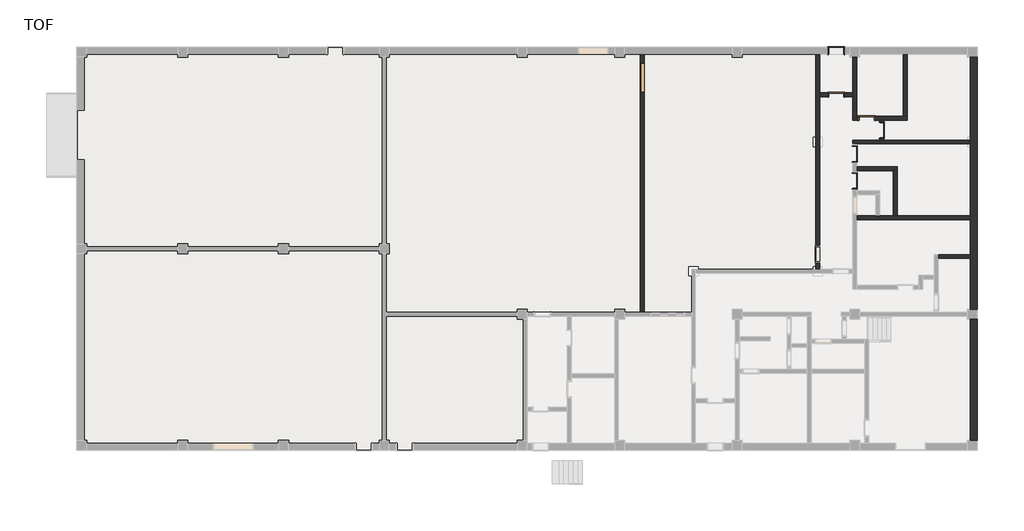
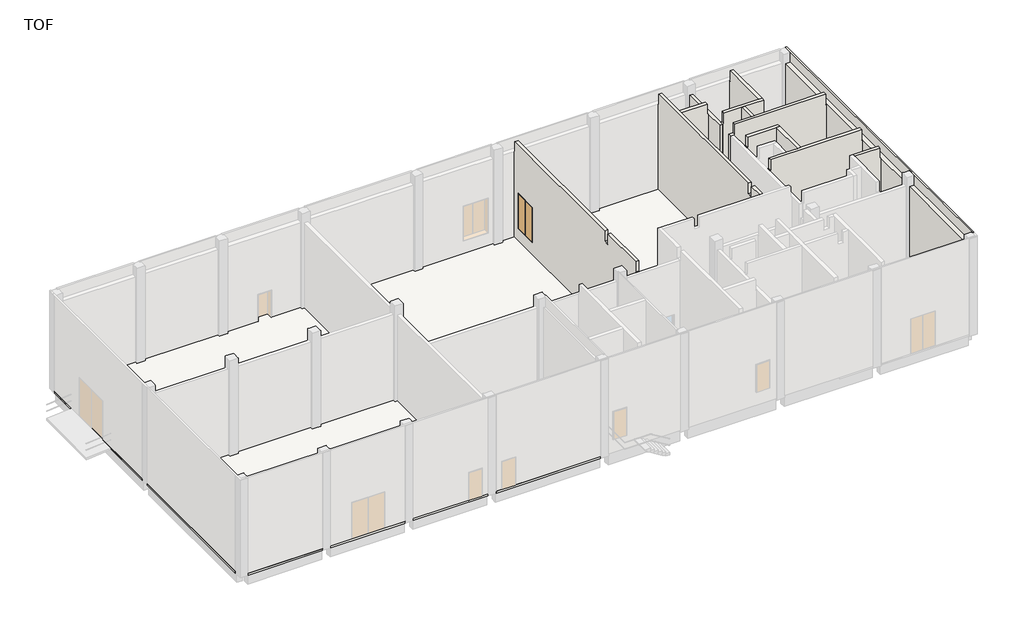
# One storey, part 3 of 5: 13 walls, 7 doors, 2 slabs.
"""IFC4 building model written with IfcOpenShell, lengths in millimetres."""

import ifcopenshell
import ifcopenshell.guid

model = None  # the IFC model being written
_history = None  # IfcOwnerHistory: only IFC2X3 demands one
_inside = {}  # id of a spatial element -> (the spatial element, [elements in it])
_under = {}  # id of a project, library or spatial element -> (it, [spatial elements below it])
_declared = {}  # id of a project -> (the project, [libraries it declares])
_typed = {}  # id of a type object -> (the type object, [elements of that type])
_made_of = {}  # id of a material, layer set ... -> (it, [elements and type objects made of it])


def new_model(schema):
    """Start an empty IFC model of exactly this schema.

    Asked for "IFC4X3", IfcOpenShell would pick the latest addendum, in which some entities
    have other attributes; the version numbers below select the first issue.
    IFC2X3 requires an IfcOwnerHistory on every rooted entity: one is made here for all.
    """
    global model, _history
    if schema == "IFC4X3":
        model = ifcopenshell.file(schema_version=(4, 3, 0, 0))
    else:
        model = ifcopenshell.file(schema=schema)
    _inside.clear()
    _under.clear()
    _declared.clear()
    _typed.clear()
    _made_of.clear()
    _history = None
    if model.schema == "IFC2X3":
        org = make("IfcOrganization", Name="unknown")
        user = make(
            "IfcPersonAndOrganization",
            ThePerson=make("IfcPerson", FamilyName="unknown"),
            TheOrganization=org,
        )
        app = make(
            "IfcApplication",
            ApplicationDeveloper=org,
            Version="unknown",
            ApplicationFullName="unknown",
            ApplicationIdentifier="unknown",
        )
        _history = make(
            "IfcOwnerHistory",
            OwningUser=user,
            OwningApplication=app,
            ChangeAction="ADDED",
            CreationDate=0,
        )
    return model


def make(cls, **values):
    """One entity of the class cls with the attributes given. An attribute that is None is left unset."""
    return model.create_entity(
        cls, **{name: value for name, value in values.items() if value is not None}
    )


def rooted(cls, **values):
    """An entity with a GlobalId (a new one), such as an element, a storey or a relation."""
    return make(cls, GlobalId=ifcopenshell.guid.new(), OwnerHistory=_history, **values)


def si_unit(unit_type, name, prefix=None):
    """IfcSIUnit, for example si_unit("LENGTHUNIT", "METRE", prefix="MILLI")."""
    return make("IfcSIUnit", UnitType=unit_type, Prefix=prefix, Name=name)


def assignment(units):
    """IfcUnitAssignment: the units of a project."""
    return None if units is None else make("IfcUnitAssignment", Units=units)


def point(xyz):
    """IfcCartesianPoint."""
    return None if xyz is None else make("IfcCartesianPoint", Coordinates=xyz)


def direction(xyz):
    """IfcDirection."""
    return None if xyz is None else make("IfcDirection", DirectionRatios=xyz)


def frame(location, z_axis=None, x_axis=None):
    """IfcAxis2Placement3D, a coordinate frame: its origin and axes. An axis left out is left unset."""
    return make(
        "IfcAxis2Placement3D",
        Location=point(location),
        Axis=direction(z_axis),
        RefDirection=direction(x_axis),
    )


def origin():
    """The frame at (0, 0, 0) with its axes left unset."""
    return frame((0.0, 0.0, 0.0))


def origin_with_axes():
    """The frame at (0, 0, 0) with the z axis (0, 0, 1) and the x axis (1, 0, 0) written out."""
    return frame((0.0, 0.0, 0.0), z_axis=(0.0, 0.0, 1.0), x_axis=(1.0, 0.0, 0.0))


def place(relative_to, where):
    """IfcLocalPlacement: puts the frame where relative to a parent placement (None: the world)."""
    return make(
        "IfcLocalPlacement", PlacementRelTo=relative_to, RelativePlacement=where
    )


def context(
    kind, dimensions, precision=None, world=None, true_north=None, identifier=None
):
    """IfcGeometricRepresentationContext, for example the 3D "Model" context."""
    return make(
        "IfcGeometricRepresentationContext",
        ContextIdentifier=identifier,
        ContextType=kind,
        CoordinateSpaceDimension=dimensions,
        Precision=precision,
        WorldCoordinateSystem=world,
        TrueNorth=true_north,
    )


def project(units=None, contexts=None):
    """IfcProject with its units and contexts."""
    return rooted(
        "IfcProject",
        Name="project",
        RepresentationContexts=contexts,
        UnitsInContext=assignment(units),
    )


def spatial(cls, under=None, at=None, **own):
    """A site, building, storey or space (cls), placed at a placement, below another one or the project."""
    s = rooted(cls, ObjectPlacement=at, **own)
    if under is not None:
        _under.setdefault(under.id(), (under, []))[1].append(s)
    return s


def polyline(points):
    """IfcPolyline through the points."""
    return make("IfcPolyline", Points=[point(p) for p in points])


def outline(outer, holes=None, kind="AREA"):
    """IfcArbitraryClosedProfileDef: a profile drawn as a closed curve; with holes, ...WithVoids."""
    if holes is None:
        return make("IfcArbitraryClosedProfileDef", ProfileType=kind, OuterCurve=outer)
    return make(
        "IfcArbitraryProfileDefWithVoids",
        ProfileType=kind,
        OuterCurve=outer,
        InnerCurves=holes,
    )


def extrude(swept, where, along, depth):
    """IfcExtrudedAreaSolid: the profile swept, set in the frame where, extruded along a direction by depth."""
    return make(
        "IfcExtrudedAreaSolid",
        SweptArea=swept,
        Position=where,
        ExtrudedDirection=direction(along),
        Depth=depth,
    )


def faces_of(points, faces, orient=None, outer=None):
    """IfcFace entities. A face is a list of loops; a loop is a list of indices into points, from 0.

    orient and outer hold one flag for each loop. By default every Orientation is true, the
    first loop of a face is its IfcFaceOuterBound and the others are IfcFaceBound.
    """
    made = []
    for i, loops in enumerate(faces):
        bounds = []
        for j, loop in enumerate(loops):
            is_outer = j == 0 if outer is None else outer[i][j]
            bounds.append(
                make(
                    "IfcFaceOuterBound" if is_outer else "IfcFaceBound",
                    Bound=make("IfcPolyLoop", Polygon=[points[k] for k in loop]),
                    Orientation=True if orient is None else orient[i][j],
                )
            )
        made.append(make("IfcFace", Bounds=bounds))
    return made


def faceted_brep(points, faces, orient=None, outer=None, voids=None):
    """IfcFacetedBrep: a solid bounded by flat faces; with voids (closed shells), ...WithVoids."""
    shared = [point(p) for p in points]
    hull = make("IfcClosedShell", CfsFaces=faces_of(shared, faces, orient, outer))
    if voids is None:
        return make("IfcFacetedBrep", Outer=hull)
    return make(
        "IfcFacetedBrepWithVoids",
        Outer=hull,
        Voids=[
            make(cls, CfsFaces=faces_of(shared, fs, o, b)) for cls, fs, o, b in voids
        ],
    )


def shape(context_of_items, identifier, shape_type, items):
    """IfcShapeRepresentation: the items that make up one representation, for example the "Body"."""
    return make(
        "IfcShapeRepresentation",
        ContextOfItems=context_of_items,
        RepresentationIdentifier=identifier,
        RepresentationType=shape_type,
        Items=items,
    )


def source(mapping_origin, context_of_items, identifier, shape_type, items):
    """IfcRepresentationMap: a shape defined once, which mapped items show again and again."""
    return make(
        "IfcRepresentationMap",
        MappingOrigin=mapping_origin,
        MappedRepresentation=shape(context_of_items, identifier, shape_type, items),
    )


def transform(
    local_origin,
    x_axis=None,
    y_axis=None,
    z_axis=None,
    scale=None,
    scale2=None,
    scale3=None,
    uniform=True,
):
    """IfcCartesianTransformationOperator3D, or its non-uniform kind. x_axis, y_axis, z_axis: its Axis1, 2, 3."""
    if uniform:
        return make(
            "IfcCartesianTransformationOperator3D",
            Axis1=direction(x_axis),
            Axis2=direction(y_axis),
            LocalOrigin=point(local_origin),
            Scale=scale,
            Axis3=direction(z_axis),
        )
    return make(
        "IfcCartesianTransformationOperator3DnonUniform",
        Axis1=direction(x_axis),
        Axis2=direction(y_axis),
        LocalOrigin=point(local_origin),
        Scale=scale,
        Axis3=direction(z_axis),
        Scale2=scale2,
        Scale3=scale3,
    )


def mapped(mapping_source, mapping_target):
    """IfcMappedItem: shows the shape of a source again, moved by a transform."""
    return make(
        "IfcMappedItem", MappingSource=mapping_source, MappingTarget=mapping_target
    )


def made_of(thing, what):
    """Note that an element or type object is made of a material, layer set ...; save() writes the relation."""
    if what is not None:
        _made_of.setdefault(what.id(), (what, []))[1].append(thing)
    return thing


def element(
    cls,
    number,
    at=None,
    inside=None,
    cuts=None,
    type_object=None,
    material=None,
    context=None,
    identifier="Body",
    shape_type=None,
    held_by="IfcProductDefinitionShape",
    body=None,
    shapes=None,
    **own,
):
    """One element of the class cls, such as IfcWall. Its Tag is "e" and its number.

    at: its placement. inside: the storey or other place that contains it. cuts: it is an
    opening in that element (IfcRelVoidsElement). A single representation is given by context,
    identifier, shape_type and body (its items); several are given by shapes. held_by: the class
    of the entity that holds the representations. save() writes the other relations.
    """
    e = rooted(cls, Tag="e%d" % number, ObjectPlacement=at, **own)
    if body is not None:
        shapes = [shape(context, identifier, shape_type, body)]
    if shapes is not None:
        e.Representation = make(held_by, Representations=shapes)
    if inside is not None:
        _inside.setdefault(inside.id(), (inside, []))[1].append(e)
    if cuts is not None:
        rooted(
            "IfcRelVoidsElement", RelatingBuildingElement=cuts, RelatedOpeningElement=e
        )
    if type_object is not None:
        _typed.setdefault(type_object.id(), (type_object, []))[1].append(e)
    return made_of(e, material)


def aggregate(whole, parts):
    """IfcRelAggregates: a whole, such as a stair, and the parts it consists of."""
    return rooted("IfcRelAggregates", RelatingObject=whole, RelatedObjects=parts)


def save(model, path):
    """Write the relations noted so far, then the file.

    IfcRelAggregates (storeys below a building ...), IfcRelContainedInSpatialStructure (elements
    in a storey), IfcRelDefinesByType, IfcRelAssociatesMaterial and IfcRelDeclares: one each for
    every whole, place, type object, material and project.
    """
    for whole, parts in _under.values():
        aggregate(whole, parts)
    for where, things in _inside.values():
        rooted(
            "IfcRelContainedInSpatialStructure",
            RelatedElements=things,
            RelatingStructure=where,
        )
    for kind, things in _typed.values():
        rooted("IfcRelDefinesByType", RelatedObjects=things, RelatingType=kind)
    for what, things in _made_of.values():
        rooted("IfcRelAssociatesMaterial", RelatedObjects=things, RelatingMaterial=what)
    for by, libraries in _declared.values():
        rooted("IfcRelDeclares", RelatingContext=by, RelatedDefinitions=libraries)
    model.write(path)


def double_door_steel_474d71af(model_context):
    return source(origin(), model_context, "Body", "SolidModel", [
        extrude(outline(polyline([(880.0, 77.0), (0.0, 77.0), (0.0, 117.0), (880.0, 117.0), (880.0, 77.0)])), frame((0.0, 0.0, 20.0), z_axis=(0.0, 0.0, 1.0), x_axis=(1.0, 0.0, 0.0)), (0.0, 0.0, 1.0), 2660.0),
        extrude(outline(polyline([(0.0, 77.0), (-880.0, 77.0), (-880.0, 117.0), (0.0, 117.0), (0.0, 77.0)])), frame((0.0, 0.0, 20.0), z_axis=(0.0, 0.0, 1.0), x_axis=(1.0, 0.0, 0.0)), (0.0, 0.0, 1.0), 2660.0),
        faceted_brep([(900.0, -117.0, 2700.0), (900.0, 117.0, 2700.0), (-900.0, 117.0, 2700.0), (-900.0, -117.0, 2700.0), (865.0, 77.0, 2665.0), (865.0, -117.0, 2665.0), (-865.0, -117.0, 2665.0), (-865.0, 77.0, 2665.0), (880.0, 117.0, 2680.0), (880.0, 77.0, 2680.0), (-880.0, 77.0, 2680.0), (-880.0, 117.0, 2680.0), (-900.0, 117.0, 0.0), (-900.0, -117.0, 0.0), (-865.0, -117.0, 35.0), (-865.0, 77.0, 35.0), (-880.0, 77.0, 20.0), (-880.0, 117.0, 20.0), (900.0, 117.0, 0.0), (880.0, 117.0, 20.0), (900.0, -117.0, 0.0), (865.0, -117.0, 35.0), (865.0, 77.0, 35.0), (880.0, 77.0, 20.0)], [[[0, 1, 2, 3]], [[4, 5, 6, 7]], [[8, 9, 10, 11]], [[3, 2, 12, 13]], [[7, 6, 14, 15]], [[11, 10, 16, 17]], [[18, 12, 2, 1], [8, 11, 17, 19]], [[13, 12, 18, 20]], [[0, 3, 13, 20], [21, 14, 6, 5]], [[15, 14, 21, 22]], [[23, 16, 10, 9], [4, 7, 15, 22]], [[17, 16, 23, 19]], [[20, 18, 1, 0]], [[22, 21, 5, 4]], [[19, 23, 9, 8]]]),
    ])


def single_door_steel_cad2a4f8(model_context):
    return source(origin(), model_context, "Body", "SolidModel", [
        extrude(outline(polyline([(470.0, -245.0), (-470.0, -245.0), (-470.0, -210.0), (470.0, -210.0), (470.0, -245.0)])), origin_with_axes(), (0.0, 0.0, 1.0), 2120.0),
        faceted_brep([(470.0, -245.0, 0.0), (470.0, -210.0, 0.0), (450.0, -210.0, 0.0), (450.0, 210.0, 0.0), (470.0, 210.0, 0.0), (470.0, 245.0, 0.0), (500.0, 245.0, 0.0), (500.0, -245.0, 0.0), (500.0, -245.0, 2150.0), (-500.0, -245.0, 2150.0), (-500.0, -245.0, 0.0), (-470.0, -245.0, 0.0), (-470.0, -245.0, 2120.0), (470.0, -245.0, 2120.0), (500.0, 245.0, 2150.0), (470.0, 245.0, 2120.0), (-470.0, 245.0, 2120.0), (-470.0, 245.0, 0.0), (-500.0, 245.0, 0.0), (-500.0, 245.0, 2150.0), (470.0, 210.0, 2120.0), (450.0, 210.0, 2100.0), (-450.0, 210.0, 2100.0), (-450.0, 210.0, 0.0), (-470.0, 210.0, 0.0), (-470.0, 210.0, 2120.0), (450.0, -210.0, 2100.0), (470.0, -210.0, 2120.0), (-470.0, -210.0, 2120.0), (-470.0, -210.0, 0.0), (-450.0, -210.0, 0.0), (-450.0, -210.0, 2100.0)], [[[0, 1, 2, 3, 4, 5, 6, 7]], [[7, 8, 9, 10, 11, 12, 13, 0]], [[6, 14, 8, 7]], [[5, 15, 16, 17, 18, 19, 14, 6]], [[4, 20, 15, 5]], [[3, 21, 22, 23, 24, 25, 20, 4]], [[2, 26, 21, 3]], [[1, 27, 28, 29, 30, 31, 26, 2]], [[0, 13, 27, 1]], [[12, 11, 29, 28]], [[11, 10, 18, 17, 24, 23, 30, 29]], [[19, 18, 10, 9]], [[25, 24, 17, 16]], [[31, 30, 23, 22]], [[14, 19, 9, 8]], [[20, 25, 16, 15]], [[26, 31, 22, 21]], [[13, 12, 28, 27]]]),
    ])


def single_door_steel_d38beafa(model_context):
    return source(origin(), model_context, "Body", "SolidModel", [
        extrude(outline(polyline([(470.0, 147.0), (470.0, 112.0), (-470.0, 112.0), (-470.0, 147.0), (470.0, 147.0)])), origin_with_axes(), (0.0, 0.0, 1.0), 2120.0),
        faceted_brep([(470.0, 147.0, 0.0), (500.0, 147.0, 0.0), (500.0, -147.0, 0.0), (470.0, -147.0, 0.0), (470.0, -112.0, 0.0), (450.0, -112.0, 0.0), (450.0, 112.0, 0.0), (470.0, 112.0, 0.0), (470.0, 147.0, 2120.0), (-470.0, 147.0, 2120.0), (-470.0, 147.0, 0.0), (-500.0, 147.0, 0.0), (-500.0, 147.0, 2150.0), (500.0, 147.0, 2150.0), (500.0, -147.0, 2150.0), (-500.0, -147.0, 2150.0), (-500.0, -147.0, 0.0), (-470.0, -147.0, 0.0), (-470.0, -147.0, 2120.0), (470.0, -147.0, 2120.0), (470.0, -112.0, 2120.0), (-470.0, -112.0, 2120.0), (-470.0, -112.0, 0.0), (-450.0, -112.0, 0.0), (-450.0, -112.0, 2100.0), (450.0, -112.0, 2100.0), (450.0, 112.0, 2100.0), (-450.0, 112.0, 2100.0), (-450.0, 112.0, 0.0), (-470.0, 112.0, 0.0), (-470.0, 112.0, 2120.0), (470.0, 112.0, 2120.0)], [[[0, 1, 2, 3, 4, 5, 6, 7]], [[1, 0, 8, 9, 10, 11, 12, 13]], [[2, 1, 13, 14]], [[3, 2, 14, 15, 16, 17, 18, 19]], [[4, 3, 19, 20]], [[5, 4, 20, 21, 22, 23, 24, 25]], [[6, 5, 25, 26]], [[7, 6, 26, 27, 28, 29, 30, 31]], [[0, 7, 31, 8]], [[9, 30, 29, 10]], [[10, 29, 28, 23, 22, 17, 16, 11]], [[15, 12, 11, 16]], [[21, 18, 17, 22]], [[27, 24, 23, 28]], [[14, 13, 12, 15]], [[20, 19, 18, 21]], [[26, 25, 24, 27]], [[8, 31, 30, 9]]]),
    ])


def single_door_steel_221a647d(model_context):
    return source(origin(), model_context, "Body", "SolidModel", [
        extrude(outline(polyline([(470.0, -147.0), (-470.0, -147.0), (-470.0, -112.0), (470.0, -112.0), (470.0, -147.0)])), origin_with_axes(), (0.0, 0.0, 1.0), 2120.0),
        faceted_brep([(470.0, -147.0, 0.0), (470.0, -112.0, 0.0), (450.0, -112.0, 0.0), (450.0, 112.0, 0.0), (470.0, 112.0, 0.0), (470.0, 147.0, 0.0), (500.0, 147.0, 0.0), (500.0, -147.0, 0.0), (500.0, -147.0, 2150.0), (-500.0, -147.0, 2150.0), (-500.0, -147.0, 0.0), (-470.0, -147.0, 0.0), (-470.0, -147.0, 2120.0), (470.0, -147.0, 2120.0), (500.0, 147.0, 2150.0), (470.0, 147.0, 2120.0), (-470.0, 147.0, 2120.0), (-470.0, 147.0, 0.0), (-500.0, 147.0, 0.0), (-500.0, 147.0, 2150.0), (470.0, 112.0, 2120.0), (450.0, 112.0, 2100.0), (-450.0, 112.0, 2100.0), (-450.0, 112.0, 0.0), (-470.0, 112.0, 0.0), (-470.0, 112.0, 2120.0), (450.0, -112.0, 2100.0), (470.0, -112.0, 2120.0), (-470.0, -112.0, 2120.0), (-470.0, -112.0, 0.0), (-450.0, -112.0, 0.0), (-450.0, -112.0, 2100.0)], [[[0, 1, 2, 3, 4, 5, 6, 7]], [[7, 8, 9, 10, 11, 12, 13, 0]], [[6, 14, 8, 7]], [[5, 15, 16, 17, 18, 19, 14, 6]], [[4, 20, 15, 5]], [[3, 21, 22, 23, 24, 25, 20, 4]], [[2, 26, 21, 3]], [[1, 27, 28, 29, 30, 31, 26, 2]], [[0, 13, 27, 1]], [[12, 11, 29, 28]], [[11, 10, 18, 17, 24, 23, 30, 29]], [[19, 18, 10, 9]], [[25, 24, 17, 16]], [[31, 30, 23, 22]], [[14, 19, 9, 8]], [[20, 25, 16, 15]], [[26, 31, 22, 21]], [[13, 12, 28, 27]]]),
    ])


model = new_model("IFC4")

# Units and contexts
model_context = context("Model", 3, world=origin())
ifc_project = project(units=[si_unit("LENGTHUNIT", "METRE", prefix="MILLI")], contexts=[model_context])

# Site, building, storey
site = spatial("IfcSite", under=ifc_project)
building = spatial("IfcBuilding", under=site)
storey = spatial("IfcBuildingStorey", under=building, Name="TOF", Elevation=150.0)

# Doors
placement = place(None, origin())
double_door_steel_shape = double_door_steel_474d71af(model_context)
element("IfcDoor", 1, ObjectType="Double Door_Steel", at=placement, inside=storey, context=model_context, shape_type="MappedRepresentation", body=[
    mapped(double_door_steel_shape, transform((33274.7, 22486.5208589, 1150.0), x_axis=(0.0, 1.0, 0.0), y_axis=(-1.0, 0.0, 0.0), z_axis=(0.0, 0.0, 1.0))),
])
single_door_steel_shape = single_door_steel_cad2a4f8(model_context)
element("IfcDoor", 2, ObjectType="Single Door_Steel", at=placement, inside=storey, context=model_context, shape_type="MappedRepresentation", body=[
    mapped(single_door_steel_shape, transform((44824.7, 24101.5208589, 1150.0), x_axis=(-1.0, 0.0, 0.0), y_axis=(0.0, -1.0, 0.0), z_axis=(0.0, 0.0, 1.0))),
])
single_door_steel_2_shape = single_door_steel_d38beafa(model_context)
element("IfcDoor", 3, ObjectType="Single Door_Steel", at=placement, inside=storey, context=model_context, shape_type="MappedRepresentation", body=[
    mapped(single_door_steel_2_shape, transform((46641.7, 20066.5208589, 1150.0), x_axis=(1.0, 0.0, 0.0), y_axis=(0.0, 1.0, 0.0), z_axis=(0.0, 0.0, 1.0))),
])
element("IfcDoor", 4, ObjectType="Single Door_Steel", at=placement, inside=storey, context=model_context, shape_type="MappedRepresentation", body=[
    mapped(single_door_steel_2_shape, transform((45924.7, 17949.5208589, 1150.0), x_axis=(0.0, -1.0, 0.0), y_axis=(1.0, 0.0, 0.0), z_axis=(0.0, 0.0, 1.0))),
])
element("IfcDoor", 5, ObjectType="Single Door_Steel", at=placement, inside=storey, context=model_context, shape_type="MappedRepresentation", body=[
    mapped(single_door_steel_2_shape, transform((45924.7, 16350.3721317, 1150.0), x_axis=(0.0, -1.0, 0.0), y_axis=(1.0, 0.0, 0.0), z_axis=(0.0, 0.0, 1.0))),
])
single_door_steel_3_shape = single_door_steel_221a647d(model_context)
element("IfcDoor", 6, ObjectType="Single Door_Steel", at=placement, inside=storey, context=model_context, shape_type="MappedRepresentation", body=[
    mapped(single_door_steel_3_shape, transform((44824.7, 21469.5208589, 1150.0), x_axis=(-1.0, 0.0, 0.0), y_axis=(0.0, -1.0, 0.0), z_axis=(0.0, 0.0, 1.0))),
])
element("IfcDoor", 7, ObjectType="Single Door_Steel", at=placement, inside=storey, context=model_context, shape_type="MappedRepresentation", body=[
    mapped(single_door_steel_3_shape, transform((47541.7, 19366.5208589, 1150.0), x_axis=(0.0, 1.0, 0.0), y_axis=(-1.0, 0.0, 0.0), z_axis=(0.0, 0.0, 1.0))),
])

# Slabs
element("IfcSlab", 8, at=placement, inside=storey, context=model_context, shape_type="Brep", body=[
    faceted_brep([(224.7, 12316.5208589, 50.0), (224.7, 12616.5208589, 50.0), (124.7, 12616.5208589, 50.0), (-275.3, 12616.5208589, 50.0), (-375.3, 12616.5208589, 50.0), (-375.3, 23716.5208589, 50.0), (-275.3, 23716.5208589, 50.0), (124.7, 23716.5208589, 50.0), (224.7, 23716.5208589, 50.0), (224.7, 23816.5208589, 50.0), (224.7, 24216.5208589, 50.0), (224.7, 24316.5208589, 50.0), (5624.7, 24316.5208589, 50.0), (5624.7, 24216.5208589, 50.0), (5624.7, 23816.5208589, 50.0), (5624.7, 23716.5208589, 50.0), (6224.7, 23716.5208589, 50.0), (6224.7, 23816.5208589, 50.0), (6224.7, 24216.5208589, 50.0), (6224.7, 24316.5208589, 50.0), (11624.7, 24316.5208589, 50.0), (11624.7, 24216.5208589, 50.0), (11624.7, 23816.5208589, 50.0), (11624.7, 23716.5208589, 50.0), (12224.7, 23716.5208589, 50.0), (12224.7, 23816.5208589, 50.0), (12224.7, 24216.5208589, 50.0), (12224.7, 24316.5208589, 50.0), (17624.7, 24316.5208589, 50.0), (17624.7, 24216.5208589, 50.0), (17624.7, 23816.5208589, 50.0), (17624.7, 23716.5208589, 50.0), (18224.7, 23716.5208589, 50.0), (18224.7, 23816.5208589, 50.0), (18224.7, 24216.5208589, 50.0), (18224.7, 24316.5208589, 50.0), (25824.7, 24316.5208589, 50.0), (25824.7, 24216.5208589, 50.0), (25824.7, 23816.5208589, 50.0), (25824.7, 23716.5208589, 50.0), (26424.7, 23716.5208589, 50.0), (26424.7, 23816.5208589, 50.0), (26424.7, 24216.5208589, 50.0), (26424.7, 24316.5208589, 50.0), (31624.7, 24316.5208589, 50.0), (31624.7, 24216.5208589, 50.0), (31624.7, 23816.5208589, 50.0), (31624.7, 23716.5208589, 50.0), (32224.7, 23716.5208589, 50.0), (32224.7, 23816.5208589, 50.0), (32224.7, 24216.5208589, 50.0), (32224.7, 24316.5208589, 50.0), (38624.7, 24316.5208589, 50.0), (38624.7, 24216.5208589, 50.0), (38624.7, 23816.5208589, 50.0), (38624.7, 23716.5208589, 50.0), (39224.7, 23716.5208589, 50.0), (39224.7, 23816.5208589, 50.0), (39224.7, 24216.5208589, 50.0), (39224.7, 24316.5208589, 50.0), (43724.7, 24316.5208589, 50.0), (43724.7, 24216.5208589, 50.0), (43724.7, 23816.5208589, 50.0), (43724.7, 18966.5208589, 50.0), (43424.7, 18966.5208589, 50.0), (43424.7, 18366.5208589, 50.0), (43724.7, 18366.5208589, 50.0), (43724.7, 11266.5208589, 50.0), (43424.7, 11266.5208589, 50.0), (43424.7, 10966.5208589, 50.0), (36624.7, 10966.5208589, 50.0), (36624.7, 11266.5208589, 50.0), (36024.7, 11266.5208589, 50.0), (36024.7, 10666.5208589, 50.0), (36324.7, 10666.5208589, 50.0), (36324.7, 8416.5208589, 50.0), (32224.7, 8416.5208589, 50.0), (32224.7, 8716.5208589, 50.0), (31624.7, 8716.5208589, 50.0), (31624.7, 8416.5208589, 50.0), (26424.7, 8416.5208589, 50.0), (26424.7, 8716.5208589, 50.0), (25824.7, 8716.5208589, 50.0), (25824.7, 8416.5208589, 50.0), (17924.7, 8416.5208589, 50.0), (17924.7, 12016.5208589, 50.0), (18224.7, 12016.5208589, 50.0), (18224.7, 12616.5208589, 50.0), (17624.7, 12616.5208589, 50.0), (17624.7, 12316.5208589, 50.0), (12224.7, 12316.5208589, 50.0), (12224.7, 12616.5208589, 50.0), (11624.7, 12616.5208589, 50.0), (11624.7, 12316.5208589, 50.0), (6224.7, 12316.5208589, 50.0), (6224.7, 12616.5208589, 50.0), (5624.7, 12616.5208589, 50.0), (5624.7, 12316.5208589, 50.0), (5624.7, 12616.5208589, 200.0), (6224.7, 12616.5208589, 200.0), (6224.7, 12433.5208589, 200.0), (11624.7, 12433.5208589, 200.0), (11624.7, 12616.5208589, 200.0), (12224.7, 12616.5208589, 200.0), (12224.7, 12433.5208589, 200.0), (17624.7, 12433.5208589, 200.0), (17624.7, 12616.5208589, 200.0), (17807.7, 12616.5208589, 200.0), (17807.7, 23716.5208589, 200.0), (17624.7, 23716.5208589, 200.0), (17624.7, 23886.5208589, 200.0), (15507.7, 23886.5208589, 200.0), (15507.7, 24316.5208589, 200.0), (14507.7, 24316.5208589, 200.0), (14507.7, 23886.5208589, 200.0), (12224.7, 23886.5208589, 200.0), (12224.7, 23716.5208589, 200.0), (11624.7, 23716.5208589, 200.0), (11624.7, 23886.5208589, 200.0), (6224.7, 23886.5208589, 200.0), (6224.7, 23716.5208589, 200.0), (5624.7, 23716.5208589, 200.0), (5624.7, 23886.5208589, 200.0), (224.7, 23886.5208589, 200.0), (224.7, 23716.5208589, 200.0), (54.7, 23716.5208589, 200.0), (54.7, 20586.5208589, 200.0), (-375.3, 20586.5208589, 200.0), (-375.3, 17586.5208589, 200.0), (54.7, 17586.5208589, 200.0), (54.7, 12616.5208589, 200.0), (224.7, 12616.5208589, 200.0), (224.7, 12433.5208589, 200.0), (5624.7, 12433.5208589, 200.0), (18224.7, 12616.5208589, 200.0), (18224.7, 12016.5208589, 200.0), (18041.7, 12016.5208589, 200.0), (18041.7, 8533.5208589, 200.0), (25824.7, 8533.5208589, 200.0), (25824.7, 8716.5208589, 200.0), (26424.7, 8716.5208589, 200.0), (26424.7, 8533.5208589, 200.0), (31624.7, 8533.5208589, 200.0), (31624.7, 8716.5208589, 200.0), (32224.7, 8716.5208589, 200.0), (32224.7, 8533.5208589, 200.0), (33157.7, 8533.5208589, 200.0), (33157.7, 23886.5208589, 200.0), (32224.7, 23886.5208589, 200.0), (32224.7, 23716.5208589, 200.0), (31624.7, 23716.5208589, 200.0), (31624.7, 23886.5208589, 200.0), (26424.7, 23886.5208589, 200.0), (26424.7, 23716.5208589, 200.0), (25824.7, 23716.5208589, 200.0), (25824.7, 23886.5208589, 200.0), (18224.7, 23886.5208589, 200.0), (18224.7, 23716.5208589, 200.0), (18041.7, 23716.5208589, 200.0), (18041.7, 12616.5208589, 200.0), (39224.7, 23716.5208589, 200.0), (38624.7, 23716.5208589, 200.0), (38624.7, 23886.5208589, 200.0), (33391.7, 23886.5208589, 200.0), (33391.7, 8533.5208589, 200.0), (36207.7, 8533.5208589, 200.0), (36207.7, 8416.5208589, 200.0), (36324.7, 8416.5208589, 200.0), (36324.7, 10666.5208589, 200.0), (36024.7, 10666.5208589, 200.0), (36024.7, 11266.5208589, 200.0), (36624.7, 11266.5208589, 200.0), (36624.7, 11083.5208589, 200.0), (43424.7, 11083.5208589, 200.0), (43424.7, 11266.5208589, 200.0), (43607.7, 11266.5208589, 200.0), (43607.7, 18366.5208589, 200.0), (43424.7, 18366.5208589, 200.0), (43424.7, 18966.5208589, 200.0), (43607.7, 18966.5208589, 200.0), (43607.7, 23886.5208589, 200.0), (39224.7, 23886.5208589, 200.0), (-375.3, 12616.5208589, 150.0), (-375.3, 17586.5208589, 150.0), (-375.3, 20586.5208589, 150.0), (-375.3, 23716.5208589, 150.0), (224.7, 24316.5208589, 150.0), (5624.7, 24316.5208589, 150.0), (6224.7, 24316.5208589, 150.0), (11624.7, 24316.5208589, 150.0), (12224.7, 24316.5208589, 150.0), (14507.7, 24316.5208589, 150.0), (15507.7, 24316.5208589, 150.0), (17624.7, 24316.5208589, 150.0), (18224.7, 24316.5208589, 150.0), (25824.7, 24316.5208589, 150.0), (26424.7, 24316.5208589, 150.0), (31624.7, 24316.5208589, 150.0), (39224.7, 24316.5208589, 150.0), (43724.7, 24316.5208589, 150.0), (32224.7, 24316.5208589, 150.0), (38624.7, 24316.5208589, 150.0), (43724.7, 18366.5208589, 150.0), (43724.7, 11266.5208589, 150.0), (43724.7, 24216.5208589, 150.0), (43724.7, 23816.5208589, 150.0), (43724.7, 18966.5208589, 150.0), (43424.7, 10966.5208589, 150.0), (36624.7, 10966.5208589, 150.0), (36207.7, 8416.5208589, 150.0), (32224.7, 8416.5208589, 150.0), (25824.7, 8416.5208589, 150.0), (17924.7, 8416.5208589, 150.0), (31624.7, 8416.5208589, 150.0), (26424.7, 8416.5208589, 150.0), (17924.7, 12016.5208589, 150.0), (5624.7, 12316.5208589, 150.0), (224.7, 12316.5208589, 150.0), (11624.7, 12316.5208589, 150.0), (6224.7, 12316.5208589, 150.0), (17624.7, 12316.5208589, 150.0), (12224.7, 12316.5208589, 150.0), (224.7, 12433.5208589, 150.0), (54.7, 12616.5208589, 150.0), (6224.7, 12433.5208589, 150.0), (5624.7, 12433.5208589, 150.0), (12224.7, 12433.5208589, 150.0), (11624.7, 12433.5208589, 150.0), (18041.7, 12016.5208589, 150.0), (17624.7, 12433.5208589, 150.0), (18041.7, 12616.5208589, 150.0), (17807.7, 12616.5208589, 150.0), (224.7, 23886.5208589, 150.0), (54.7, 23716.5208589, 150.0), (6224.7, 23886.5208589, 150.0), (5624.7, 23886.5208589, 150.0), (12224.7, 23886.5208589, 150.0), (11624.7, 23886.5208589, 150.0), (18224.7, 23886.5208589, 150.0), (17807.7, 23716.5208589, 150.0), (18041.7, 23716.5208589, 150.0), (17624.7, 23886.5208589, 150.0), (26424.7, 23886.5208589, 150.0), (25824.7, 23886.5208589, 150.0), (32224.7, 23886.5208589, 150.0), (31624.7, 23886.5208589, 150.0), (39224.7, 23886.5208589, 150.0), (38624.7, 23886.5208589, 150.0), (26424.7, 8533.5208589, 150.0), (25824.7, 8533.5208589, 150.0), (32224.7, 8533.5208589, 150.0), (31624.7, 8533.5208589, 150.0), (36624.7, 11083.5208589, 150.0), (43424.7, 11083.5208589, 150.0), (43607.7, 11266.5208589, 150.0), (43607.7, 18366.5208589, 150.0), (43607.7, 18966.5208589, 150.0), (33157.7, 23886.5208589, 150.0), (43607.7, 23886.5208589, 150.0), (33391.7, 23886.5208589, 150.0), (15507.7, 23886.5208589, 150.0), (14507.7, 23886.5208589, 150.0), (18041.7, 8533.5208589, 150.0), (33157.7, 8533.5208589, 150.0), (36207.7, 8533.5208589, 150.0), (33391.7, 8533.5208589, 150.0), (54.7, 20586.5208589, 150.0), (54.7, 17586.5208589, 150.0)], [[[0, 1, 2, 3, 4, 5, 6, 7, 8, 9, 10, 11, 12, 13, 14, 15, 16, 17, 18, 19, 20, 21, 22, 23, 24, 25, 26, 27, 28, 29, 30, 31, 32, 33, 34, 35, 36, 37, 38, 39, 40, 41, 42, 43, 44, 45, 46, 47, 48, 49, 50, 51, 52, 53, 54, 55, 56, 57, 58, 59, 60, 61, 62, 63, 64, 65, 66, 67, 68, 69, 70, 71, 72, 73, 74, 75, 76, 77, 78, 79, 80, 81, 82, 83, 84, 85, 86, 87, 88, 89, 90, 91, 92, 93, 94, 95, 96, 97]], [[98, 99, 100, 101, 102, 103, 104, 105, 106, 107, 108, 109, 110, 111, 112, 113, 114, 115, 116, 117, 118, 119, 120, 121, 122, 123, 124, 125, 126, 127, 128, 129, 130, 131, 132, 133]], [[134, 135, 136, 137, 138, 139, 140, 141, 142, 143, 144, 145, 146, 147, 148, 149, 150, 151, 152, 153, 154, 155, 156, 157, 158, 159]], [[160, 161, 162, 163, 164, 165, 166, 167, 168, 169, 170, 171, 172, 173, 174, 175, 176, 177, 178, 179, 180, 181]], [[5, 4, 182, 183, 128, 127, 184, 185]], [[12, 11, 186, 187]], [[20, 19, 188, 189]], [[28, 27, 190, 191, 113, 112, 192, 193]], [[36, 35, 194, 195]], [[44, 43, 196, 197]], [[60, 59, 198, 199]], [[52, 51, 200, 201]], [[67, 66, 202, 203]], [[63, 62, 61, 60, 199, 204, 205, 206]], [[70, 69, 207, 208]], [[167, 75, 74, 168]], [[75, 167, 166, 209, 210, 76]], [[84, 83, 211, 212]], [[80, 79, 213, 214]], [[85, 84, 212, 215]], [[0, 97, 216, 217]], [[94, 93, 218, 219]], [[90, 89, 220, 221]], [[1, 0, 217, 222, 132, 131]], [[4, 3, 2, 1, 131, 130, 223, 182]], [[95, 94, 219, 224, 100, 99]], [[97, 96, 98, 133, 225, 216]], [[96, 95, 99, 98]], [[91, 90, 221, 226, 104, 103]], [[93, 92, 102, 101, 227, 218]], [[92, 91, 103, 102]], [[87, 86, 135, 134]], [[86, 85, 215, 228, 136, 135]], [[89, 88, 106, 105, 229, 220]], [[88, 87, 134, 159, 230, 231, 107, 106]], [[11, 10, 9, 8, 124, 123, 232, 186]], [[8, 7, 6, 5, 185, 233, 125, 124]], [[19, 18, 17, 16, 120, 119, 234, 188]], [[16, 15, 121, 120]], [[15, 14, 13, 12, 187, 235, 122, 121]], [[27, 26, 25, 24, 116, 115, 236, 190]], [[24, 23, 117, 116]], [[23, 22, 21, 20, 189, 237, 118, 117]], [[35, 34, 33, 32, 157, 156, 238, 194]], [[32, 31, 109, 108, 239, 240, 158, 157]], [[31, 30, 29, 28, 193, 241, 110, 109]], [[43, 42, 41, 40, 153, 152, 242, 196]], [[40, 39, 154, 153]], [[39, 38, 37, 36, 195, 243, 155, 154]], [[51, 50, 49, 48, 149, 148, 244, 200]], [[48, 47, 150, 149]], [[47, 46, 45, 44, 197, 245, 151, 150]], [[59, 58, 57, 56, 160, 181, 246, 198]], [[56, 55, 161, 160]], [[55, 54, 53, 52, 201, 247, 162, 161]], [[81, 80, 214, 248, 141, 140]], [[83, 82, 139, 138, 249, 211]], [[82, 81, 140, 139]], [[77, 76, 210, 250, 145, 144]], [[79, 78, 143, 142, 251, 213]], [[78, 77, 144, 143]], [[171, 71, 70, 208, 252, 172]], [[73, 169, 168, 74]], [[169, 73, 72, 170]], [[170, 72, 71, 171]], [[68, 174, 173, 253, 207, 69]], [[174, 68, 67, 203, 254, 175]], [[65, 177, 176, 255, 202, 66]], [[177, 65, 64, 178]], [[178, 64, 63, 206, 256, 179]], [[244, 148, 147, 257]], [[246, 181, 180, 258]], [[162, 247, 259, 163]], [[241, 260, 111, 110]], [[243, 238, 156, 155]], [[245, 242, 152, 151]], [[235, 232, 123, 122]], [[237, 234, 119, 118]], [[114, 261, 236, 115]], [[215, 212, 211, 249, 262, 228]], [[199, 198, 246, 258, 256, 206, 205, 204]], [[201, 200, 244, 257, 263, 250, 210, 209, 264, 265, 259, 247]], [[238, 243, 195, 194]], [[242, 245, 197, 196]], [[232, 235, 187, 186]], [[234, 237, 189, 188]], [[261, 191, 190, 236]], [[192, 260, 241, 193]], [[239, 231, 230, 240]], [[251, 248, 214, 213]], [[255, 254, 203, 202]], [[191, 261, 114, 113]], [[260, 192, 112, 111]], [[233, 266, 126, 125]], [[129, 267, 223, 130]], [[184, 266, 233, 185]], [[267, 183, 182, 223]], [[266, 184, 127, 126]], [[183, 267, 129, 128]], [[222, 225, 133, 132]], [[224, 227, 101, 100]], [[226, 229, 105, 104]], [[225, 222, 217, 216]], [[227, 224, 219, 218]], [[229, 226, 221, 220]], [[231, 239, 108, 107]], [[136, 228, 262, 137]], [[240, 230, 159, 158]], [[263, 257, 147, 146]], [[259, 265, 164, 163]], [[265, 264, 165, 164]], [[262, 249, 138, 137]], [[250, 263, 146, 145]], [[248, 251, 142, 141]], [[165, 264, 209, 166]], [[252, 253, 173, 172]], [[253, 252, 208, 207]], [[254, 255, 176, 175]], [[256, 258, 180, 179]]]),
])
element("IfcSlab", 9, at=placement, inside=storey, context=model_context, shape_type="Brep", body=[
    faceted_brep([(224.7, 12016.5208589, 0.0), (224.7, 12316.5208589, 0.0), (5624.7, 12316.5208589, 0.0), (5624.7, 12016.5208589, 0.0), (6224.7, 12016.5208589, 0.0), (6224.7, 12316.5208589, 0.0), (11624.7, 12316.5208589, 0.0), (11624.7, 12016.5208589, 0.0), (12224.7, 12016.5208589, 0.0), (12224.7, 12316.5208589, 0.0), (17624.7, 12316.5208589, 0.0), (17624.7, 12016.5208589, 0.0), (17924.7, 12016.5208589, 0.0), (17924.7, 8416.5208589, 0.0), (25824.7, 8416.5208589, 0.0), (25824.7, 8116.5208589, 0.0), (26307.7, 8116.5208589, 0.0), (26307.7, 916.5208589, 0.0), (25824.7, 916.5208589, 0.0), (25824.7, 816.5208589, 0.0), (25824.7, 416.5208589, 0.0), (25824.7, 316.5208589, 0.0), (18224.7, 316.5208589, 0.0), (18224.7, 416.5208589, 0.0), (18224.7, 816.5208589, 0.0), (18224.7, 916.5208589, 0.0), (17624.7, 916.5208589, 0.0), (17624.7, 816.5208589, 0.0), (17624.7, 416.5208589, 0.0), (17624.7, 316.5208589, 0.0), (12224.7, 316.5208589, 0.0), (12224.7, 416.5208589, 0.0), (12224.7, 816.5208589, 0.0), (12224.7, 916.5208589, 0.0), (11624.7, 916.5208589, 0.0), (11624.7, 816.5208589, 0.0), (11624.7, 416.5208589, 0.0), (11624.7, 316.5208589, 0.0), (6224.7, 316.5208589, 0.0), (6224.7, 416.5208589, 0.0), (6224.7, 816.5208589, 0.0), (6224.7, 916.5208589, 0.0), (5624.7, 916.5208589, 0.0), (5624.7, 816.5208589, 0.0), (5624.7, 416.5208589, 0.0), (5624.7, 316.5208589, 0.0), (224.7, 316.5208589, 0.0), (224.7, 416.5208589, 0.0), (224.7, 816.5208589, 0.0), (224.7, 916.5208589, 0.0), (124.7, 916.5208589, 0.0), (-275.3, 916.5208589, 0.0), (-375.3, 916.5208589, 0.0), (-375.3, 12016.5208589, 0.0), (-275.3, 12016.5208589, 0.0), (124.7, 12016.5208589, 0.0), (224.7, 12316.5208589, 150.0), (224.7, 12199.5208589, 150.0), (224.7, 12016.5208589, 150.0), (54.7, 12016.5208589, 150.0), (-375.3, 12016.5208589, 150.0), (-375.3, 916.5208589, 150.0), (54.7, 916.5208589, 150.0), (224.7, 916.5208589, 150.0), (224.7, 746.5208589, 150.0), (224.7, 316.5208589, 150.0), (5624.7, 316.5208589, 150.0), (5624.7, 746.5208589, 150.0), (5624.7, 916.5208589, 150.0), (6224.7, 916.5208589, 150.0), (6224.7, 746.5208589, 150.0), (6224.7, 316.5208589, 150.0), (7731.2, 316.5208589, 150.0), (10131.2, 316.5208589, 150.0), (11624.7, 316.5208589, 150.0), (11624.7, 746.5208589, 150.0), (11624.7, 916.5208589, 150.0), (12224.7, 916.5208589, 150.0), (12224.7, 746.5208589, 150.0), (12224.7, 316.5208589, 150.0), (16207.7, 316.5208589, 150.0), (17207.7, 316.5208589, 150.0), (17624.7, 316.5208589, 150.0), (17624.7, 746.5208589, 150.0), (17624.7, 916.5208589, 150.0), (17807.7, 916.5208589, 150.0), (18041.7, 916.5208589, 150.0), (18224.7, 916.5208589, 150.0), (18224.7, 746.5208589, 150.0), (18224.7, 316.5208589, 150.0), (18641.7, 316.5208589, 150.0), (19641.7, 316.5208589, 150.0), (25824.7, 316.5208589, 150.0), (25824.7, 746.5208589, 150.0), (25824.7, 916.5208589, 150.0), (26190.7, 916.5208589, 150.0), (26307.7, 916.5208589, 150.0), (26307.7, 8116.5208589, 150.0), (26190.7, 8116.5208589, 150.0), (25824.7, 8116.5208589, 150.0), (25824.7, 8299.5208589, 150.0), (25824.7, 8416.5208589, 150.0), (17924.7, 8416.5208589, 150.0), (17924.7, 12016.5208589, 150.0), (17807.7, 12016.5208589, 150.0), (17624.7, 12016.5208589, 150.0), (17624.7, 12199.5208589, 150.0), (17624.7, 12316.5208589, 150.0), (12224.7, 12316.5208589, 150.0), (12224.7, 12199.5208589, 150.0), (12224.7, 12016.5208589, 150.0), (11624.7, 12016.5208589, 150.0), (11624.7, 12199.5208589, 150.0), (11624.7, 12316.5208589, 150.0), (6224.7, 12316.5208589, 150.0), (6224.7, 12199.5208589, 150.0), (6224.7, 12016.5208589, 150.0), (5624.7, 12016.5208589, 150.0), (5624.7, 12199.5208589, 150.0), (5624.7, 12316.5208589, 150.0)], [[[0, 1, 2, 3, 4, 5, 6, 7, 8, 9, 10, 11, 12, 13, 14, 15, 16, 17, 18, 19, 20, 21, 22, 23, 24, 25, 26, 27, 28, 29, 30, 31, 32, 33, 34, 35, 36, 37, 38, 39, 40, 41, 42, 43, 44, 45, 46, 47, 48, 49, 50, 51, 52, 53, 54, 55]], [[56, 57, 58, 59, 60, 61, 62, 63, 64, 65, 66, 67, 68, 69, 70, 71, 72, 73, 74, 75, 76, 77, 78, 79, 80, 81, 82, 83, 84, 85, 86, 87, 88, 89, 90, 91, 92, 93, 94, 95, 96, 97, 98, 99, 100, 101, 102, 103, 104, 105, 106, 107, 108, 109, 110, 111, 112, 113, 114, 115, 116, 117, 118, 119]], [[102, 13, 12, 103]], [[13, 102, 101, 14]], [[16, 97, 96, 17]], [[65, 46, 45, 66]], [[71, 38, 37, 74, 73, 72]], [[79, 30, 29, 82, 81, 80]], [[89, 22, 21, 92, 91, 90]], [[60, 53, 52, 61]], [[1, 56, 119, 2]], [[5, 114, 113, 6]], [[9, 108, 107, 10]], [[0, 58, 57, 56, 1]], [[58, 0, 55, 54, 53, 60, 59]], [[4, 116, 115, 114, 5]], [[116, 4, 3, 117]], [[117, 3, 2, 119, 118]], [[8, 110, 109, 108, 9]], [[110, 8, 7, 111]], [[111, 7, 6, 113, 112]], [[11, 105, 104, 103, 12]], [[105, 11, 10, 107, 106]], [[15, 99, 98, 97, 16]], [[99, 15, 14, 101, 100]], [[63, 49, 48, 47, 46, 65, 64]], [[49, 63, 62, 61, 52, 51, 50]], [[69, 41, 40, 39, 38, 71, 70]], [[42, 68, 67, 66, 45, 44, 43]], [[68, 42, 41, 69]], [[77, 33, 32, 31, 30, 79, 78]], [[34, 76, 75, 74, 37, 36, 35]], [[76, 34, 33, 77]], [[87, 25, 24, 23, 22, 89, 88]], [[26, 84, 83, 82, 29, 28, 27]], [[84, 26, 25, 87, 86, 85]], [[18, 94, 93, 92, 21, 20, 19]], [[94, 18, 17, 96, 95]]]),
])

# Walls
element("IfcWall", 10, at=placement, inside=storey, context=model_context, shape_type="Brep", body=[
    faceted_brep([(52794.7, 18366.5208589, 150.0), (52794.7, 8716.5208589, 150.0), (52794.7, 8716.5208589, 1000.0), (52794.7, 8716.5208589, 1150.0), (52794.7, 8716.5208589, 6750.0), (52794.7, 11733.5208589, 6750.0), (52794.7, 11967.5208589, 6750.0), (52794.7, 14049.5208589, 6750.0), (52794.7, 14283.5208589, 6750.0), (52794.7, 18549.5208589, 6750.0), (52794.7, 18783.5208589, 6750.0), (52794.7, 23716.5208589, 6750.0), (52794.7, 23716.5208589, 1150.0), (52794.7, 23716.5208589, 1000.0), (52794.7, 23716.5208589, 150.0), (52794.7, 18966.5208589, 150.0), (52794.7, 18966.5208589, 1000.0), (52794.7, 18966.5208589, 1150.0), (52794.7, 18783.5208589, 1150.0), (52794.7, 18549.5208589, 1150.0), (52794.7, 18366.5208589, 1150.0), (52794.7, 18366.5208589, 1000.0), (52794.7, 8116.5208589, 150.0), (52794.7, 916.5208589, 150.0), (52794.7, 916.5208589, 200.0), (52794.7, 916.5208589, 6750.0), (52794.7, 8116.5208589, 6750.0), (52794.7, 8116.5208589, 200.0), (53224.7, 23716.5208589, 150.0), (53224.7, 23716.5208589, 7500.0), (53224.7, 24316.5208589, 7500.0), (53224.7, 24316.5208589, 7549.0), (53224.7, 746.5208589, 7549.0), (53224.7, 746.5208589, 7500.0), (53224.7, 916.5208589, 7500.0), (53224.7, 916.5208589, 150.0), (53224.7, 8116.5208589, 150.0), (53224.7, 8116.5208589, 7500.0), (53224.7, 8716.5208589, 7500.0), (53224.7, 8716.5208589, 150.0), (53224.7, 18366.5208589, 150.0), (53224.7, 18366.5208589, 1150.0), (53224.7, 18966.5208589, 1150.0), (53224.7, 18966.5208589, 150.0), (53124.7, 23716.5208589, 150.0), (53124.7, 18966.5208589, 150.0), (53124.7, 8716.5208589, 150.0), (53124.7, 18366.5208589, 150.0), (53124.7, 24316.5208589, 7500.0), (53124.7, 24316.5208589, 7549.0), (53124.7, 746.5208589, 7500.0), (53124.7, 746.5208589, 7549.0), (53124.7, 23716.5208589, 6750.0), (53124.7, 23716.5208589, 7500.0), (53124.7, 8116.5208589, 6750.0), (53124.7, 8116.5208589, 7500.0), (53124.7, 8716.5208589, 7500.0), (53124.7, 8716.5208589, 6750.0), (53124.7, 8216.5208589, 7500.0), (53124.7, 8616.5208589, 7500.0), (53124.7, 916.5208589, 7500.0), (53124.7, 916.5208589, 6750.0), (53124.7, 816.5208589, 7500.0), (53124.7, 12116.5208589, 6750.0), (53124.7, 12516.5208589, 6750.0), (53124.7, 816.5208589, 7549.0), (53124.7, 8216.5208589, 7549.0), (53124.7, 8616.5208589, 7549.0), (53124.7, 12116.5208589, 7549.0), (53124.7, 12516.5208589, 7549.0)], [[[0, 1, 2, 3, 4, 5, 6, 7, 8, 9, 10, 11, 12, 13, 14, 15, 16, 17, 18, 19, 20, 21]], [[22, 23, 24, 25, 26, 27]], [[28, 29, 30, 31, 32, 33, 34, 35, 36, 37, 38, 39, 40, 41, 42, 43]], [[14, 44, 28, 43, 45, 15]], [[39, 46, 1, 0, 47, 40]], [[22, 36, 35, 23]], [[30, 48, 49, 31]], [[50, 33, 32, 51]], [[29, 28, 44, 14, 13, 12, 11, 52, 53]], [[30, 29, 53, 48]], [[37, 36, 22, 27, 26, 54, 55]], [[39, 38, 56, 57, 4, 3, 2, 1, 46]], [[38, 37, 55, 58, 59, 56]], [[35, 34, 60, 61, 25, 24, 23]], [[34, 33, 50, 62, 60]], [[20, 41, 40, 47, 0, 21]], [[42, 17, 16, 15, 45, 43]], [[41, 20, 19, 18, 17, 42]], [[4, 57, 63, 64, 52, 11, 10, 9, 8, 7, 6, 5]], [[54, 61, 60, 62, 50, 51, 65, 66, 67, 68, 69, 49, 48, 53, 52, 64, 63, 57, 56, 59, 58, 55]], [[61, 54, 26, 25]], [[32, 31, 49, 69, 68, 67, 66, 65, 51]]]),
])
element("IfcWall", 11, at=placement, inside=storey, context=model_context, shape_type="Brep", body=[
    faceted_brep([(33157.7, 23886.5208589, 150.0), (33157.7, 8533.5208589, 150.0), (33157.7, 8533.5208589, 200.0), (33157.7, 8533.5208589, 6750.0), (33157.7, 8616.5208589, 6750.0), (33157.7, 8616.5208589, 7549.0), (33157.7, 12116.5208589, 7549.0), (33157.7, 12116.5208589, 6750.0), (33157.7, 12516.5208589, 6750.0), (33157.7, 12516.5208589, 7549.0), (33157.7, 23816.5208589, 7549.0), (33157.7, 23816.5208589, 6750.0), (33157.7, 23886.5208589, 6750.0), (33157.7, 23886.5208589, 200.0), (33157.7, 23386.5208589, 1150.0), (33157.7, 23386.5208589, 3850.0), (33157.7, 21586.5208589, 3850.0), (33157.7, 21586.5208589, 1150.0), (33391.7, 8533.5208589, 150.0), (33391.7, 23886.5208589, 150.0), (33391.7, 23886.5208589, 200.0), (33391.7, 23886.5208589, 6750.0), (33391.7, 23816.5208589, 6750.0), (33391.7, 23816.5208589, 7549.0), (33391.7, 12516.5208589, 7549.0), (33391.7, 12516.5208589, 6750.0), (33391.7, 12116.5208589, 6750.0), (33391.7, 12116.5208589, 7549.0), (33391.7, 8616.5208589, 7549.0), (33391.7, 8616.5208589, 6750.0), (33391.7, 8533.5208589, 6750.0), (33391.7, 8533.5208589, 200.0), (33391.7, 23386.5208589, 3850.0), (33391.7, 23386.5208589, 1150.0), (33391.7, 21586.5208589, 1150.0), (33391.7, 21586.5208589, 3850.0)], [[[0, 1, 2, 3, 4, 5, 6, 7, 8, 9, 10, 11, 12, 13], [14, 15, 16, 17]], [[18, 19, 20, 21, 22, 23, 24, 25, 26, 27, 28, 29, 30, 31], [32, 33, 34, 35]], [[1, 0, 19, 18]], [[19, 0, 13, 12, 21, 20]], [[1, 18, 31, 30, 3, 2]], [[14, 33, 32, 15]], [[15, 32, 35, 16]], [[34, 17, 16, 35]], [[33, 14, 17, 34]], [[26, 7, 6, 27]], [[7, 26, 25, 8]], [[8, 25, 24, 9]], [[22, 11, 10, 23]], [[11, 22, 21, 12]], [[29, 4, 3, 30]], [[4, 29, 28, 5]], [[6, 5, 28, 27]], [[10, 9, 24, 23]]]),
])
element("IfcWall", 12, at=placement, inside=storey, context=model_context, shape_type="Brep", body=[
    faceted_brep([(43841.7, 11266.5208589, 1150.0), (43841.7, 11266.5208589, 1000.0), (43841.7, 11266.5208589, 150.0), (43841.7, 18366.5208589, 150.0), (43841.7, 18366.5208589, 1000.0), (43841.7, 18366.5208589, 1150.0), (43841.7, 18966.5208589, 1150.0), (43841.7, 18966.5208589, 1000.0), (43841.7, 18966.5208589, 150.0), (43841.7, 23886.5208589, 150.0), (43841.7, 23886.5208589, 1000.0), (43841.7, 23886.5208589, 1150.0), (43841.7, 23886.5208589, 6750.0), (43841.7, 23816.5208589, 6750.0), (43841.7, 23816.5208589, 7549.0), (43841.7, 21586.5208589, 7549.0), (43841.7, 21352.5208589, 7549.0), (43841.7, 12516.5208589, 7549.0), (43841.7, 12516.5208589, 6750.0), (43841.7, 12116.5208589, 6750.0), (43841.7, 12116.5208589, 7549.0), (43841.7, 11083.5208589, 7549.0), (43841.7, 11083.5208589, 1150.0), (43841.7, 12483.5208589, 3300.0), (43841.7, 12483.5208589, 1150.0), (43841.7, 11483.5208589, 1150.0), (43841.7, 11483.5208589, 3300.0), (43607.7, 11266.5208589, 150.0), (43607.7, 11266.5208589, 200.0), (43607.7, 11266.5208589, 1150.0), (43607.7, 11083.5208589, 1150.0), (43607.7, 11083.5208589, 7549.0), (43607.7, 12116.5208589, 7549.0), (43607.7, 12116.5208589, 6750.0), (43607.7, 12516.5208589, 6750.0), (43607.7, 12516.5208589, 7549.0), (43607.7, 23816.5208589, 7549.0), (43607.7, 23816.5208589, 6750.0), (43607.7, 23886.5208589, 6750.0), (43607.7, 23886.5208589, 200.0), (43607.7, 23886.5208589, 150.0), (43607.7, 18966.5208589, 150.0), (43607.7, 18966.5208589, 200.0), (43607.7, 18966.5208589, 1150.0), (43607.7, 18366.5208589, 1150.0), (43607.7, 18366.5208589, 200.0), (43607.7, 18366.5208589, 150.0), (43607.7, 12483.5208589, 1150.0), (43607.7, 12483.5208589, 3300.0), (43607.7, 11483.5208589, 3300.0), (43607.7, 11483.5208589, 1150.0), (43724.7, 18966.5208589, 150.0), (43724.7, 11266.5208589, 150.0), (43724.7, 18366.5208589, 150.0)], [[[0, 1, 2, 3, 4, 5, 6, 7, 8, 9, 10, 11, 12, 13, 14, 15, 16, 17, 18, 19, 20, 21, 22], [23, 24, 25, 26]], [[27, 28, 29, 30, 31, 32, 33, 34, 35, 36, 37, 38, 39, 40, 41, 42, 43, 44, 45, 46], [47, 48, 49, 50]], [[40, 9, 8, 51, 41]], [[2, 52, 27, 46, 53, 3]], [[9, 40, 39, 38, 12, 11, 10]], [[30, 22, 21, 31]], [[47, 24, 23, 48]], [[48, 23, 26, 49]], [[25, 50, 49, 26]], [[24, 47, 50, 25]], [[0, 29, 28, 27, 52, 2, 1]], [[29, 0, 22, 30]], [[44, 5, 4, 3, 53, 46, 45]], [[6, 43, 42, 41, 51, 8, 7]], [[5, 44, 43, 6]], [[19, 33, 32, 20]], [[33, 19, 18, 34]], [[34, 18, 17, 35]], [[13, 37, 36, 14]], [[37, 13, 12, 38]], [[21, 20, 32, 31]], [[17, 16, 15, 14, 36, 35]]]),
])
element("IfcWall", 13, at=placement, inside=storey, context=model_context, shape_type="SweptSolid", body=[
    extrude(outline(polyline([(1150.0, 43841.7), (1150.0, 44324.7), (3300.0, 44324.7), (3300.0, 45324.7), (1150.0, 45324.7), (1150.0, 45807.7), (6750.0, 45807.7), (6750.0, 45724.7), (7549.0, 45724.7), (7549.0, 43841.7), (1150.0, 43841.7)])), frame((0.0, 21352.5208589, 0.0), z_axis=(0.0, 1.0, 0.0), x_axis=(0.0, 0.0, 1.0)), (0.0, 0.0, 1.0), 234.0),
])
element("IfcWall", 14, at=placement, inside=storey, context=model_context, shape_type="Brep", body=[
    faceted_brep([(45807.7, 23716.5208589, 1150.0), (45807.7, 21586.5208589, 1150.0), (45807.7, 21352.5208589, 1150.0), (45807.7, 19949.5208589, 1150.0), (45807.7, 19949.5208589, 6750.0), (45807.7, 21352.5208589, 6750.0), (45807.7, 21586.5208589, 6750.0), (45807.7, 23716.5208589, 6750.0), (46041.7, 19949.5208589, 1150.0), (46041.7, 20183.5208589, 1150.0), (46041.7, 23716.5208589, 1150.0), (46041.7, 23716.5208589, 6750.0), (46041.7, 20183.5208589, 6750.0), (46041.7, 19949.5208589, 6750.0)], [[[0, 1, 2, 3, 4, 5, 6, 7]], [[8, 9, 10, 11, 12, 13]], [[8, 3, 2, 1, 0, 10, 9]], [[3, 8, 13, 4]], [[10, 0, 7, 11]], [[7, 6, 5, 4, 13, 12, 11]]]),
])
element("IfcWall", 15, at=placement, inside=storey, context=model_context, shape_type="Brep", body=[
    faceted_brep([(50894.7, 11733.5208589, 1150.0), (52794.7, 11733.5208589, 1150.0), (52794.7, 11733.5208589, 6750.0), (52724.7, 11733.5208589, 6750.0), (52724.7, 11733.5208589, 7549.0), (50894.7, 11733.5208589, 7549.0), (52794.7, 11967.5208589, 1150.0), (50894.7, 11967.5208589, 1150.0), (50894.7, 11967.5208589, 7549.0), (52724.7, 11967.5208589, 7549.0), (52724.7, 11967.5208589, 6750.0), (52794.7, 11967.5208589, 6750.0), (50894.7, 11850.5208589, 1150.0), (52794.7, 11850.5208589, 1150.0)], [[[0, 1, 2, 3, 4, 5]], [[6, 7, 8, 9, 10, 11]], [[1, 0, 12, 7, 6, 13]], [[7, 12, 0, 5, 8]], [[1, 13, 6, 11, 2]], [[10, 3, 2, 11]], [[3, 10, 9, 4]], [[5, 4, 9, 8]]]),
])
element("IfcWall", 16, at=placement, inside=storey, context=model_context, shape_type="Brep", body=[
    faceted_brep([(45807.7, 18549.5208589, 1150.0), (46041.7, 18549.5208589, 1150.0), (52794.7, 18549.5208589, 1150.0), (52794.7, 18549.5208589, 6750.0), (52724.7, 18549.5208589, 6750.0), (52724.7, 18549.5208589, 7549.0), (46124.7, 18549.5208589, 7549.0), (46124.7, 18549.5208589, 6750.0), (46041.7, 18549.5208589, 6750.0), (45807.7, 18549.5208589, 6750.0), (52794.7, 18783.5208589, 1150.0), (47658.7, 18783.5208589, 1150.0), (47424.7, 18783.5208589, 1150.0), (45807.7, 18783.5208589, 1150.0), (45807.7, 18783.5208589, 6750.0), (46124.7, 18783.5208589, 6750.0), (46124.7, 18783.5208589, 7549.0), (47424.7, 18783.5208589, 7549.0), (47658.7, 18783.5208589, 7549.0), (52724.7, 18783.5208589, 7549.0), (52724.7, 18783.5208589, 6750.0), (52794.7, 18783.5208589, 6750.0)], [[[0, 1, 2, 3, 4, 5, 6, 7, 8, 9]], [[10, 11, 12, 13, 14, 15, 16, 17, 18, 19, 20, 21]], [[2, 1, 0, 13, 12, 11, 10]], [[2, 10, 21, 3]], [[13, 0, 9, 14]], [[15, 7, 6, 16]], [[7, 15, 14, 9, 8]], [[20, 4, 3, 21]], [[4, 20, 19, 5]], [[6, 5, 19, 18, 17, 16]]]),
])
element("IfcWall", 17, at=placement, inside=storey, context=model_context, shape_type="Brep", body=[
    faceted_brep([(47141.7, 19949.5208589, 1150.0), (47424.7, 19949.5208589, 1150.0), (47658.7, 19949.5208589, 1150.0), (49041.7, 19949.5208589, 1150.0), (49041.7, 19949.5208589, 7549.0), (47658.7, 19949.5208589, 7549.0), (47424.7, 19949.5208589, 7549.0), (46124.7, 19949.5208589, 7549.0), (46124.7, 19949.5208589, 6750.0), (46041.7, 19949.5208589, 6750.0), (46041.7, 19949.5208589, 1150.0), (46141.7, 19949.5208589, 1150.0), (46141.7, 19949.5208589, 3300.0), (47141.7, 19949.5208589, 3300.0), (49041.7, 20183.5208589, 1150.0), (48807.7, 20183.5208589, 1150.0), (47141.7, 20183.5208589, 1150.0), (47141.7, 20183.5208589, 3300.0), (46141.7, 20183.5208589, 3300.0), (46141.7, 20183.5208589, 1150.0), (46041.7, 20183.5208589, 1150.0), (46041.7, 20183.5208589, 6750.0), (46124.7, 20183.5208589, 6750.0), (46124.7, 20183.5208589, 7549.0), (48807.7, 20183.5208589, 7549.0), (49041.7, 20183.5208589, 7549.0)], [[[0, 1, 2, 3, 4, 5, 6, 7, 8, 9, 10, 11, 12, 13]], [[14, 15, 16, 17, 18, 19, 20, 21, 22, 23, 24, 25]], [[14, 3, 2, 1, 0, 16, 15]], [[10, 20, 19, 11]], [[3, 14, 25, 4]], [[20, 10, 9, 21]], [[13, 17, 16, 0]], [[17, 13, 12, 18]], [[18, 12, 11, 19]], [[22, 8, 7, 23]], [[8, 22, 21, 9]], [[7, 6, 5, 4, 25, 24, 23]]]),
])
element("IfcWall", 18, at=placement, inside=storey, context=model_context, shape_type="SweptSolid", body=[
    extrude(outline(polyline([(23886.5208589, 1150.0), (20183.5208589, 1150.0), (20183.5208589, 7549.0), (23816.5208589, 7549.0), (23816.5208589, 6750.0), (23886.5208589, 6750.0), (23886.5208589, 1150.0)])), frame((48807.7, 0.0, 0.0), z_axis=(1.0, 0.0, 0.0), x_axis=(0.0, 1.0, 0.0)), (0.0, 0.0, 1.0), 234.0),
])
element("IfcWall", 19, at=placement, inside=storey, context=model_context, shape_type="SweptSolid", body=[
    extrude(outline(polyline([(19949.5208589, 1150.0), (19866.5208589, 1150.0), (19866.5208589, 3300.0), (18866.5208589, 3300.0), (18866.5208589, 1150.0), (18783.5208589, 1150.0), (18783.5208589, 7549.0), (19949.5208589, 7549.0), (19949.5208589, 1150.0)])), frame((47424.7, 0.0, 0.0), z_axis=(1.0, 0.0, 0.0), x_axis=(0.0, 1.0, 0.0)), (0.0, 0.0, 1.0), 234.0),
])
element("IfcWall", 20, at=placement, inside=storey, context=model_context, shape_type="Brep", body=[
    faceted_brep([(46041.7, 14049.5208589, 1150.0), (52794.7, 14049.5208589, 1150.0), (52794.7, 14049.5208589, 6750.0), (52724.7, 14049.5208589, 6750.0), (52724.7, 14049.5208589, 7549.0), (46124.7, 14049.5208589, 7549.0), (46124.7, 14049.5208589, 6750.0), (46041.7, 14049.5208589, 6750.0), (52794.7, 14283.5208589, 1150.0), (48441.7, 14283.5208589, 1150.0), (48207.7, 14283.5208589, 1150.0), (47401.7, 14283.5208589, 1150.0), (47167.7, 14283.5208589, 1150.0), (46041.7, 14283.5208589, 1150.0), (46041.7, 14283.5208589, 6750.0), (46124.7, 14283.5208589, 6750.0), (46124.7, 14283.5208589, 7549.0), (47167.7, 14283.5208589, 7549.0), (47401.7, 14283.5208589, 7549.0), (48207.7, 14283.5208589, 7549.0), (48441.7, 14283.5208589, 7549.0), (52724.7, 14283.5208589, 7549.0), (52724.7, 14283.5208589, 6750.0), (52794.7, 14283.5208589, 6750.0)], [[[0, 1, 2, 3, 4, 5, 6, 7]], [[8, 9, 10, 11, 12, 13, 14, 15, 16, 17, 18, 19, 20, 21, 22, 23]], [[1, 0, 13, 12, 11, 10, 9, 8]], [[1, 8, 23, 2]], [[13, 0, 7, 14]], [[15, 6, 5, 16]], [[6, 15, 14, 7]], [[22, 3, 2, 23]], [[3, 22, 21, 4]], [[5, 4, 21, 20, 19, 18, 17, 16]]]),
])
element("IfcWall", 21, at=placement, inside=storey, context=model_context, shape_type="Brep", body=[
    faceted_brep([(46041.7, 16946.5208589, 1150.0), (48207.7, 16946.5208589, 1150.0), (48441.7, 16946.5208589, 1150.0), (48441.7, 16946.5208589, 7549.0), (48207.7, 16946.5208589, 7549.0), (46124.7, 16946.5208589, 7549.0), (46124.7, 16946.5208589, 6750.0), (46041.7, 16946.5208589, 6750.0), (48441.7, 17180.5208589, 1150.0), (46041.7, 17180.5208589, 1150.0), (46041.7, 17180.5208589, 6750.0), (46124.7, 17180.5208589, 6750.0), (46124.7, 17180.5208589, 7549.0), (48441.7, 17180.5208589, 7549.0)], [[[0, 1, 2, 3, 4, 5, 6, 7]], [[8, 9, 10, 11, 12, 13]], [[2, 1, 0, 9, 8]], [[9, 0, 7, 10]], [[2, 8, 13, 3]], [[11, 6, 5, 12]], [[6, 11, 10, 7]], [[5, 4, 3, 13, 12]]]),
])
element("IfcWall", 22, at=placement, inside=storey, context=model_context, shape_type="SweptSolid", body=[
    extrude(outline(polyline([(48207.7, 14283.5208589), (48207.7, 16946.5208589), (48441.7, 16946.5208589), (48441.7, 14283.5208589), (48207.7, 14283.5208589)])), frame((0.0, 0.0, 1150.0), z_axis=(0.0, 0.0, 1.0), x_axis=(1.0, 0.0, 0.0)), (0.0, 0.0, 1.0), 6399.0),
])

save(model, "model.ifc")
